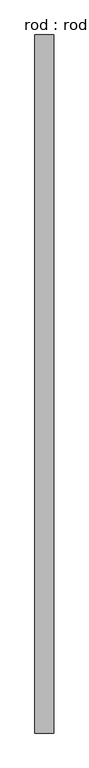
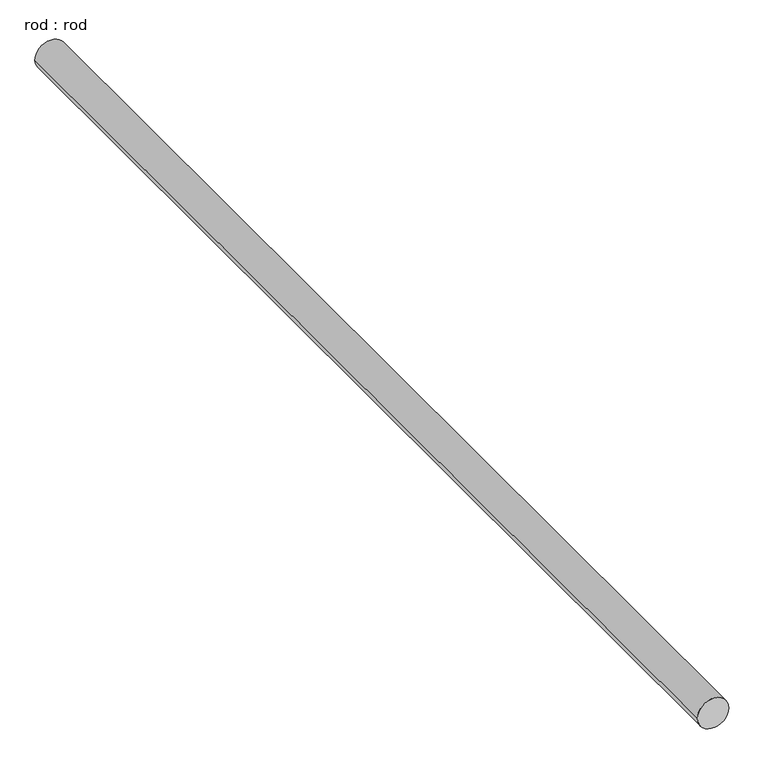
"""IFC4 building model written with IfcOpenShell, lengths in millimetres: proxy geometry, rod : rod."""

from ifc_helpers import new_model, si_unit, point, frame, frame_2d, origin, place, context, project, spatial, circle_curve, trimmed, segment, composite_curve, outline, extrude, source, transform, mapped, element, save


def rod_rod_6dd04e5c(model_context):
    return source(origin(), model_context, "Body", "SweptSolid", [
        extrude(outline(composite_curve([segment(trimmed(circle_curve(frame_2d((0.0108462, 0.0)), 200.0), [point((0.0108462, 200.0))], [point((0.0108462, -200.0))], False, "CARTESIAN"), True, "CONTINUOUS"), segment(trimmed(circle_curve(frame_2d((0.0108462, 0.0)), 200.0), [point((0.0108462, -200.0))], [point((0.0108462, 200.0))], False, "CARTESIAN"), True, "CONTINUOUS")], self_intersect=False)), frame((0.0, -3243.6806315, 0.0), z_axis=(0.0, 1.0, 0.0), x_axis=(0.0, 0.0, 1.0)), (0.0, 0.0, 1.0), 14672.8184938),
    ])


if __name__ == "__main__":
    model = new_model("IFC4")
    model_context = context("Model", 3, world=origin())
    ifc_project = project(units=[si_unit("LENGTHUNIT", "METRE", prefix="MILLI")], contexts=[model_context])
    site = spatial("IfcSite", under=ifc_project)
    building = spatial("IfcBuilding", under=site)
    placement = place(None, origin())
    rod_rod_shape = rod_rod_6dd04e5c(model_context)
    element("IfcBuildingElementProxy", 1, Name="rod : rod", ObjectType="rod : rod", at=placement, inside=building, context=model_context, shape_type="MappedRepresentation", body=[
        mapped(rod_rod_shape, transform((0.0, 0.0, 0.0), x_axis=(1.0, 0.0, 0.0), y_axis=(0.0, 1.0, 0.0), z_axis=(0.0, 0.0, 1.0))),
    ])
    save(model, "model.ifc")

# Revit data of these elements
# Type "rod : rod"
#   Default Elevation = 0
